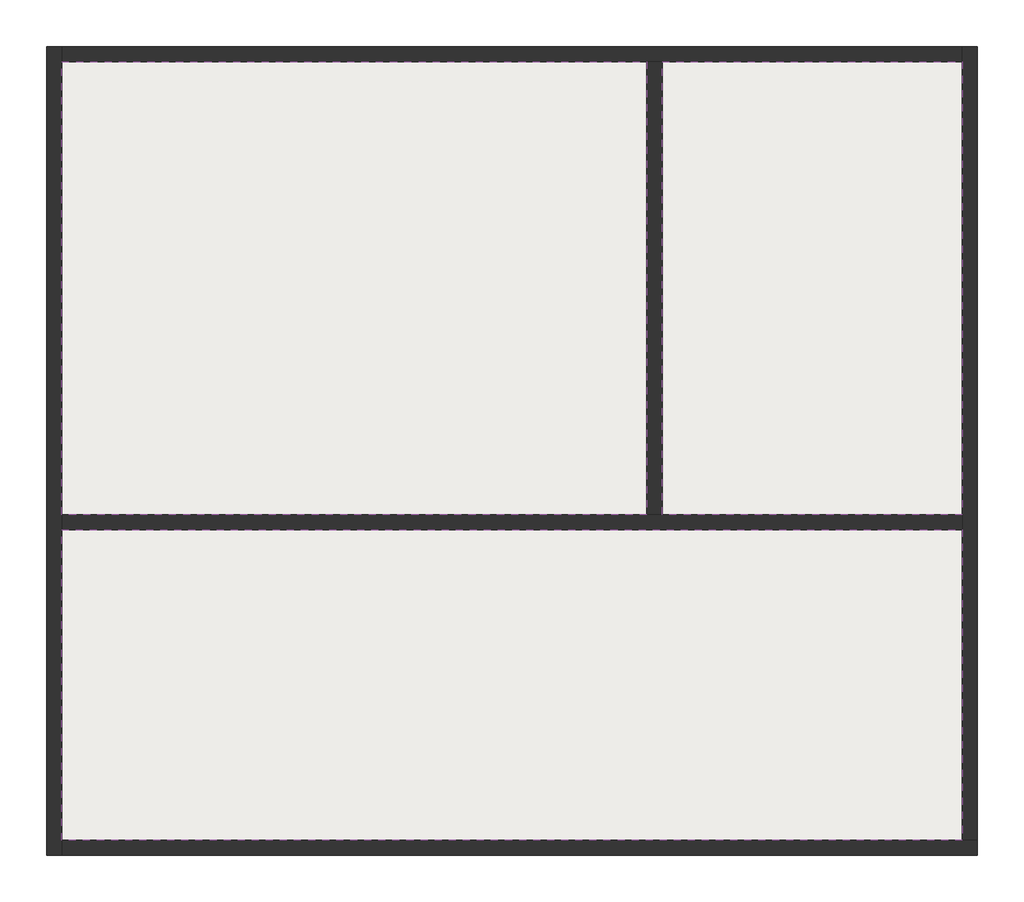
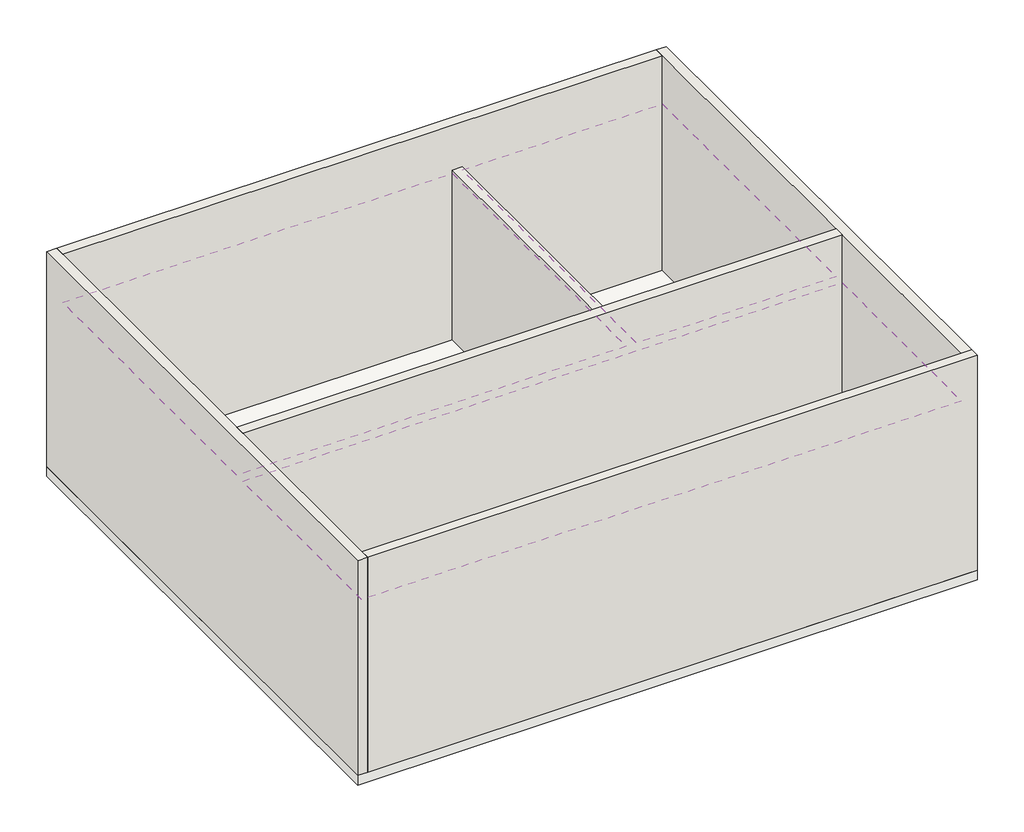
# One storey: 6 walls, 3 coverings, 1 slab.
"""IFC4 building model written with IfcOpenShell, lengths in millimetres."""

from ifc_helpers import new_model, si_unit, frame, origin, place, context, project, spatial, polyline, outline, extrude, faceted_brep, element, save

model = new_model("IFC4")

# Units and contexts
model_context = context("Model", 3, world=origin())
ifc_project = project(units=[si_unit("LENGTHUNIT", "METRE", prefix="MILLI")], contexts=[model_context])

# Site, building, storey
site = spatial("IfcSite", under=ifc_project)
building = spatial("IfcBuilding", under=site)
storey = spatial("IfcBuildingStorey", under=building, Name="レベル 1", Elevation=500.0)

# Coverings
placement = place(None, origin())
element("IfcCovering", 1, ObjectType="グリッド 600x600mm", at=placement, inside=storey, context=model_context, shape_type="SweptSolid", body=[
    extrude(outline(polyline([(-4139.1497645, -1548.6940898), (-9889.1497645, -1548.6940898), (-9889.1497645, 2901.3059102), (-4139.1497645, 2901.3059102), (-4139.1497645, -1548.6940898)])), frame((0.0, 0.0, 3100.0), z_axis=(0.0, 0.0, 1.0), x_axis=(1.0, 0.0, 0.0)), (0.0, 0.0, 1.0), 52.0),
])
element("IfcCovering", 2, ObjectType="グリッド 600x600mm", at=placement, inside=storey, context=model_context, shape_type="SweptSolid", body=[
    extrude(outline(polyline([(-1039.1497645, 2901.3059102), (-1039.1497645, -1548.6940898), (-3989.1497645, -1548.6940898), (-3989.1497645, 2901.3059102), (-1039.1497645, 2901.3059102)])), frame((0.0, 0.0, 3100.0), z_axis=(0.0, 0.0, 1.0), x_axis=(1.0, 0.0, 0.0)), (0.0, 0.0, 1.0), 52.0),
])
element("IfcCovering", 3, ObjectType="グリッド 600x600mm", at=placement, inside=storey, context=model_context, shape_type="SweptSolid", body=[
    extrude(outline(polyline([(-1039.1497645, -4748.6940898), (-9889.1497645, -4748.6940898), (-9889.1497645, -1698.6940898), (-1039.1497645, -1698.6940898), (-1039.1497645, -4748.6940898)])), frame((0.0, 0.0, 3100.0), z_axis=(0.0, 0.0, 1.0), x_axis=(1.0, 0.0, 0.0)), (0.0, 0.0, 1.0), 52.0),
])

# Slab
element("IfcSlab", 4, ObjectType="一般 150 mm", at=placement, inside=storey, context=model_context, shape_type="SweptSolid", body=[
    extrude(outline(polyline([(-889.1497645, 3051.3059102), (-889.1497645, -4898.6940898), (-10039.1497645, -4898.6940898), (-10039.1497645, 3051.3059102), (-889.1497645, 3051.3059102)])), frame((0.0, 0.0, 350.0), z_axis=(0.0, 0.0, 1.0), x_axis=(1.0, 0.0, 0.0)), (0.0, 0.0, 1.0), 150.0),
])

# Walls
element("IfcWall", 5, ObjectType="標準-150mm", at=placement, inside=storey, context=model_context, shape_type="Brep", body=[
    faceted_brep([(-10039.1497645, 3051.3059102, 500.0), (-10039.1497645, -4898.6940898, 500.0), (-10039.1497645, -4898.6940898, 3850.0), (-10039.1497645, 3051.3059102, 3850.0), (-9889.1497645, 3051.3059102, 500.0), (-9889.1497645, 3051.3059102, 3850.0), (-9889.1497645, 2901.3059102, 3850.0), (-9889.1497645, -1548.6940898, 3850.0), (-9889.1497645, -1698.6940898, 3850.0), (-9889.1497645, -4748.6940898, 3850.0), (-9889.1497645, -4898.6940898, 3850.0), (-9889.1497645, -4898.6940898, 500.0), (-9889.1497645, -4748.6940898, 500.0), (-9889.1497645, -1698.6940898, 500.0), (-9889.1497645, -1548.6940898, 500.0), (-9889.1497645, 2901.3059102, 500.0)], [[[0, 1, 2, 3]], [[4, 5, 6, 7, 8, 9, 10, 11, 12, 13, 14, 15]], [[1, 0, 4, 15, 14, 13, 12, 11]], [[3, 2, 10, 9, 8, 7, 6, 5]], [[0, 3, 5, 4]], [[2, 1, 11, 10]]]),
])
element("IfcWall", 6, ObjectType="標準-150mm", at=placement, inside=storey, context=model_context, shape_type="Brep", body=[
    faceted_brep([(-9889.1497645, -1698.6940898, 500.0), (-1039.1497645, -1698.6940898, 500.0), (-1039.1497645, -1698.6940898, 3850.0), (-9889.1497645, -1698.6940898, 3850.0), (-9889.1497645, -1548.6940898, 500.0), (-9889.1497645, -1548.6940898, 3850.0), (-1039.1497645, -1548.6940898, 3850.0), (-1039.1497645, -1548.6940898, 500.0), (-3989.1497645, -1548.6940898, 500.0), (-4139.1497645, -1548.6940898, 500.0)], [[[0, 1, 2, 3]], [[4, 5, 6, 7, 8, 9]], [[1, 0, 4, 9, 8, 7]], [[0, 3, 5, 4]], [[2, 1, 7, 6]], [[3, 2, 6, 5]]]),
])
element("IfcWall", 7, ObjectType="標準-150mm", at=placement, inside=storey, context=model_context, shape_type="Brep", body=[
    faceted_brep([(-889.1497645, -4748.6940898, 500.0), (-889.1497645, 3051.3059102, 500.0), (-889.1497645, 3051.3059102, 3850.0), (-889.1497645, -4748.6940898, 3850.0), (-1039.1497645, -4748.6940898, 500.0), (-1039.1497645, -4748.6940898, 3850.0), (-1039.1497645, -1698.6940898, 3850.0), (-1039.1497645, -1548.6940898, 3850.0), (-1039.1497645, 2901.3059102, 3850.0), (-1039.1497645, 3051.3059102, 3850.0), (-1039.1497645, 3051.3059102, 500.0), (-1039.1497645, 2901.3059102, 500.0), (-1039.1497645, -1548.6940898, 500.0), (-1039.1497645, -1698.6940898, 500.0)], [[[0, 1, 2, 3]], [[4, 5, 6, 7, 8, 9, 10, 11, 12, 13]], [[1, 0, 4, 13, 12, 11, 10]], [[3, 2, 9, 8, 7, 6, 5]], [[2, 1, 10, 9]], [[0, 3, 5, 4]]]),
])
element("IfcWall", 8, ObjectType="標準-150mm", at=placement, inside=storey, context=model_context, shape_type="Brep", body=[
    faceted_brep([(-1039.1497645, 3051.3059102, 500.0), (-9889.1497645, 3051.3059102, 500.0), (-9889.1497645, 3051.3059102, 3850.0), (-1039.1497645, 3051.3059102, 3850.0), (-1039.1497645, 2901.3059102, 500.0), (-1039.1497645, 2901.3059102, 3850.0), (-9889.1497645, 2901.3059102, 3850.0), (-9889.1497645, 2901.3059102, 500.0), (-4139.1497645, 2901.3059102, 500.0), (-3989.1497645, 2901.3059102, 500.0)], [[[0, 1, 2, 3]], [[4, 5, 6, 7, 8, 9]], [[1, 0, 4, 9, 8, 7]], [[3, 2, 6, 5]], [[2, 1, 7, 6]], [[0, 3, 5, 4]]]),
])
element("IfcWall", 9, ObjectType="標準-150mm", at=placement, inside=storey, context=model_context, shape_type="SweptSolid", body=[
    extrude(outline(polyline([(-4139.1497645, -1548.6940898), (-4139.1497645, 2901.3059102), (-3989.1497645, 2901.3059102), (-3989.1497645, -1548.6940898), (-4139.1497645, -1548.6940898)])), frame((0.0, 0.0, 500.0), z_axis=(0.0, 0.0, 1.0), x_axis=(1.0, 0.0, 0.0)), (0.0, 0.0, 1.0), 2652.0),
])
element("IfcWall", 10, ObjectType="標準-150mm", at=placement, inside=storey, context=model_context, shape_type="Brep", body=[
    faceted_brep([(-9889.1497645, -4898.6940898, 500.0), (-889.1497645, -4898.6940898, 500.0), (-889.1497645, -4898.6940898, 3850.0), (-9889.1497645, -4898.6940898, 3850.0), (-9889.1497645, -4748.6940898, 500.0), (-9889.1497645, -4748.6940898, 3850.0), (-1039.1497645, -4748.6940898, 3850.0), (-889.1497645, -4748.6940898, 3850.0), (-889.1497645, -4748.6940898, 500.0), (-1039.1497645, -4748.6940898, 500.0)], [[[0, 1, 2, 3]], [[4, 5, 6, 7, 8, 9]], [[1, 0, 4, 9, 8]], [[3, 2, 7, 6, 5]], [[0, 3, 5, 4]], [[2, 1, 8, 7]]]),
])

save(model, "model.ifc")

# Revit data of these elements
# Project information
#   プロジェクト発行日 = "発行日"
#   プロジェクト ステータス = "プロジェクト ステータス"
#   クライアント名 = "オーナ"
#   計画地住所 = "ここにアドレスを入力"
#   プロジェクト名 = "プロジェクト名"
#   プロジェクト番号 = "0001"
# Type "グリッド 600x600mm"
#   built-in parameter 1002203 = 1 (stored number, unit not read)
#   built-in parameter 1002202 = 1 (stored number, unit not read)
#   Layers, outside or top first: 36 mm no material (function 1); 16 mm "天井タイル 600 x 600" (function 5)
# Type "一般 150 mm"
#   Function = 0
#   Layers, outside or top first: 150 mm no material (function 1)
# Type "標準-150mm"
#   Layers, outside or top first: 150 mm no material (function 1)
# Elements 1, 2, 3 (IfcCovering, "グリッド 600x600mm")
#   Height Offset From Level = 2600 mm
#   Phase Created = 新しい建設
#   Materials on its faces: "天井タイル 600 x 600"
# Element 4 (IfcSlab, "一般 150 mm")
#   Height Offset From Level = 0 mm
#   Phase Created = 新しい建設
# Elements 5, 6, 7, 8, 10 (IfcWall, "標準-150mm")
#   Top Offset = 0 mm
#   Base Offset = 0 mm
#   wall height = 3350 mm
#   Phase Created = 新しい建設
#   Base Constraint = レベル 1
#   Top Constraint = レベル 2
#   Materials on its faces: "既定の壁"
# Element 9 (IfcWall, "標準-150mm")
#   Top Offset = -848 mm
#   Base Offset = 0 mm
#   wall height = 2652 mm
#   Phase Created = 新しい建設
#   Base Constraint = レベル 1
#   Top Constraint = レベル 2
#   Materials on its faces: "既定の壁"
# Materials
#   "天井タイル 600 x 600": class "一般", colour RGB 235 235 235, transparency 0, Description = "吸音天井タイル", Cost = 0
#   "既定の壁": class "その他", colour RGB 127 127 127, transparency 0, Cost = 0
